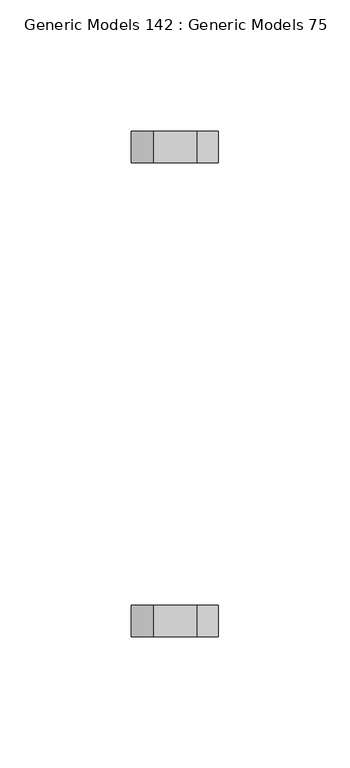
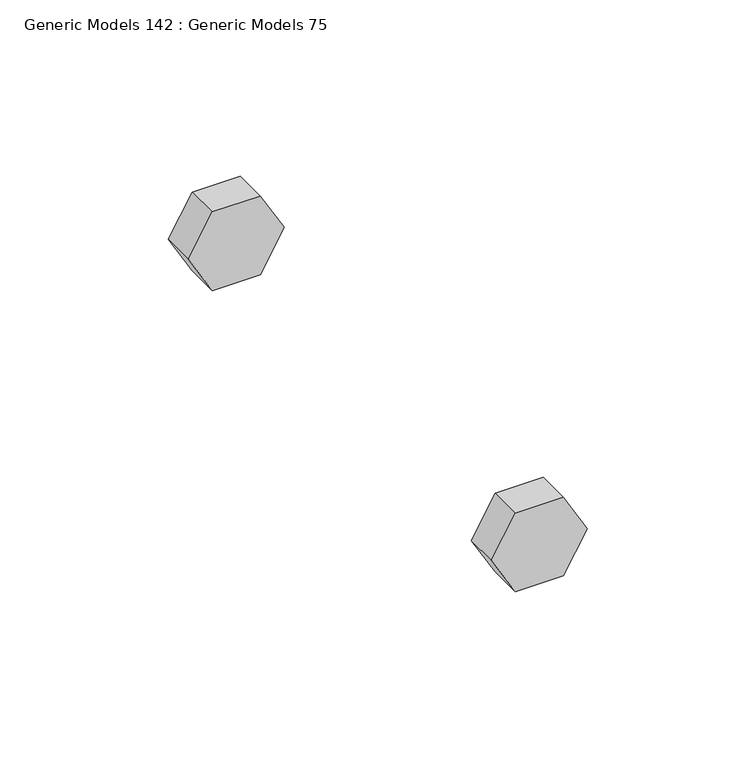
"""IFC4 building model written with IfcOpenShell, lengths in millimetres: proxy geometry, Generic Models 142 : Generic Models 75."""

from ifc_helpers import new_model, si_unit, frame, origin, place, context, project, spatial, polyline, outline, extrude, source, transform, mapped, element, save


def generic_models_142_generic_models_75_680a847f(model_context):
    return source(origin(), model_context, "Body", "SweptSolid", [
        extrude(outline(polyline([(271581.5625, 31979.8726858), (271581.5625, 31996.3704698), (271595.85, 32004.6193618), (271610.1375, 31996.3704698), (271610.1375, 31979.8726858), (271595.85, 31971.6237939), (271581.5625, 31979.8726858)])), frame((0.0, 36311.3770442, 0.0), z_axis=(0.0, 1.0, 0.0), x_axis=(0.0, 0.0, 1.0)), (0.0, 0.0, 1.0), 11.90625),
        extrude(outline(polyline([(271581.5625, 31979.8726858), (271581.5625, 31996.3704698), (271595.85, 32004.6193618), (271610.1375, 31996.3704698), (271610.1375, 31979.8726858), (271595.85, 31971.6237939), (271581.5625, 31979.8726858)])), frame((0.0, 36491.5582942, 0.0), z_axis=(0.0, 1.0, 0.0), x_axis=(0.0, 0.0, 1.0)), (0.0, 0.0, 1.0), 11.90625),
    ])


if __name__ == "__main__":
    model = new_model("IFC4")
    model_context = context("Model", 3, world=origin())
    ifc_project = project(units=[si_unit("LENGTHUNIT", "METRE", prefix="MILLI")], contexts=[model_context])
    site = spatial("IfcSite", under=ifc_project)
    building = spatial("IfcBuilding", under=site)
    placement = place(None, origin())
    generic_models_142_generic_models_75_shape = generic_models_142_generic_models_75_680a847f(model_context)
    element("IfcBuildingElementProxy", 1, Name="Generic Models 142 : Generic Models 75", ObjectType="Generic Models 142 : Generic Models 75", at=placement, inside=building, context=model_context, shape_type="MappedRepresentation", body=[
        mapped(generic_models_142_generic_models_75_shape, transform((0.0, 0.0, 0.0), x_axis=(1.0, 0.0, 0.0), y_axis=(0.0, 1.0, 0.0), z_axis=(0.0, 0.0, 1.0))),
    ])
    save(model, "model.ifc")

# Revit data of these elements
# Element 1 (IfcBuildingElementProxy, "Generic Models 142 : Generic Models 75")
#   Materials on its faces: "3/4\" GALV. THRU BOLTS"
# Materials
#   "3/4\" GALV. THRU BOLTS": class "Generic", colour RGB 105 69 171, transparency 0, Cost = 0
